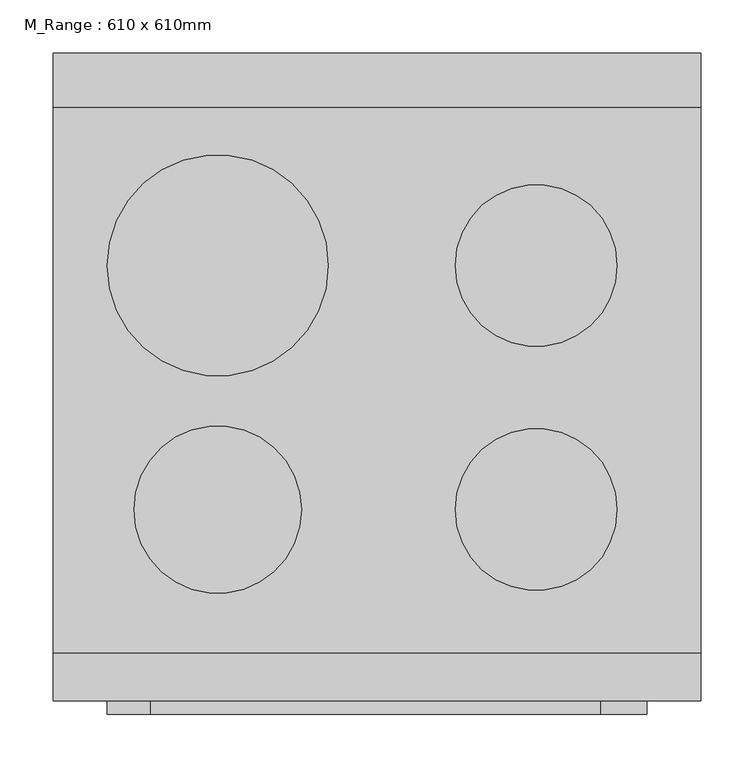
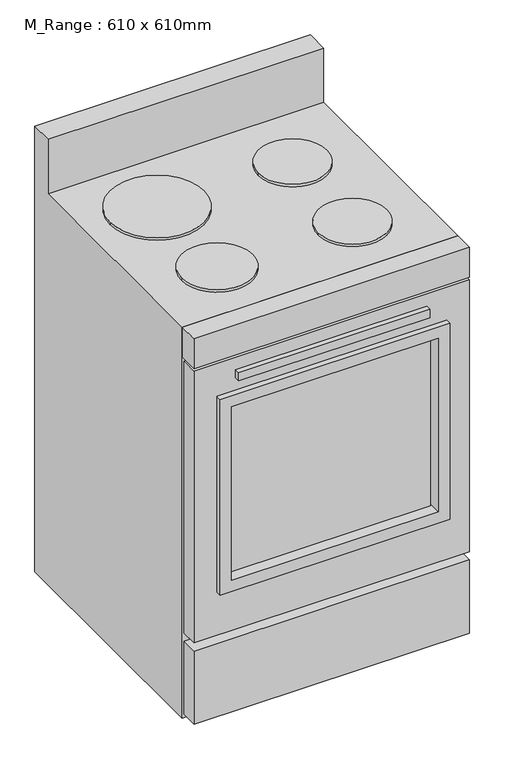
"""IFC4 building model written with IfcOpenShell, lengths in millimetres: proxy geometry, M_Range : 610 x 610mm."""

from ifc_helpers import new_model, si_unit, point, frame, frame_2d, origin, place, context, project, spatial, polyline, circle_curve, trimmed, segment, composite_curve, outline, extrude, faceted_brep, source, transform, mapped, element, save


def m_range_610_x_610mm_0f77da38(model_context):
    return source(origin(), model_context, "Body", "SolidModel", [
        faceted_brep([(610.0, 610.0, 1041.4), (610.0, 559.2, 1041.4), (610.0, 559.2, 914.4), (610.0, 45.0, 914.4), (610.0, 45.0, 0.0), (610.0, 610.0, 0.0), (0.0, 559.2, 914.4), (0.0, 559.2, 1041.4), (0.0, 610.0, 1041.4), (0.0, 610.0, 0.0), (0.0, 45.0, 0.0), (0.0, 45.0, 914.4), (584.6, 45.0, 889.2220355), (584.6, 45.0, 254.0), (25.4, 45.0, 254.0), (25.4, 45.0, 889.2220355), (25.4, 584.6, 889.2220355), (584.6, 584.6, 889.2220355), (25.4, 584.6, 254.0), (584.6, 584.6, 254.0)], [[[0, 1, 2, 3, 4, 5]], [[6, 7, 8, 9, 10, 11]], [[8, 0, 5, 9]], [[1, 0, 8, 7]], [[2, 1, 7, 6]], [[3, 11, 10, 4], [12, 13, 14, 15]], [[9, 5, 4, 10]], [[11, 3, 2, 6]], [[12, 15, 16, 17]], [[15, 14, 18, 16]], [[14, 13, 19, 18]], [[13, 12, 17, 19]], [[17, 16, 18, 19]]]),
        extrude(outline(polyline([(515.325, -12.7), (91.687309, -12.7), (91.687309, 0.0), (515.325, 0.0), (515.325, -12.7)])), frame((0.0, 0.0, 791.2768639), z_axis=(0.0, 0.0, 1.0), x_axis=(1.0, 0.0, 0.0)), (0.0, 0.0, 1.0), 19.05),
        extrude(outline(polyline([(531.2, 12.7), (76.2, 12.7), (76.2, 19.05), (531.2, 19.05), (531.2, 12.7)])), frame((0.0, 0.0, 330.2), z_axis=(0.0, 0.0, 1.0), x_axis=(1.0, 0.0, 0.0)), (0.0, 0.0, 1.0), 406.4),
        extrude(outline(polyline([(610.0, 0.0), (0.0, 0.0), (0.0, 45.0), (610.0, 45.0), (610.0, 0.0)])), frame((0.0, 0.0, 844.7720355), z_axis=(0.0, 0.0, 1.0), x_axis=(1.0, 0.0, 0.0)), (0.0, 0.0, 1.0), 69.6279645),
        extrude(outline(polyline([(762.0, 559.2), (762.0, 50.8), (304.8, 50.8), (304.8, 559.2), (762.0, 559.2)]), holes=[polyline([(736.6, 533.8), (330.2, 533.8), (330.2, 76.2), (736.6, 76.2), (736.6, 533.8)])]), frame((0.0, -12.7, 0.0), z_axis=(0.0, 1.0, 0.0), x_axis=(0.0, 0.0, 1.0)), (0.0, 0.0, 1.0), 38.1),
        extrude(outline(composite_curve([segment(trimmed(circle_curve(frame_2d((155.0, 410.0)), 104.2), [point((50.8, 410.0))], [point((259.2, 410.0))], False, "CARTESIAN"), True, "CONTINUOUS"), segment(trimmed(circle_curve(frame_2d((155.0, 410.0)), 104.2), [point((259.2, 410.0))], [point((50.8, 410.0))], False, "CARTESIAN"), True, "CONTINUOUS")], self_intersect=False)), frame((0.0, 0.0, 914.4), z_axis=(0.0, 0.0, 1.0), x_axis=(1.0, 0.0, 0.0)), (0.0, 0.0, 1.0), 6.35),
        extrude(outline(composite_curve([segment(trimmed(circle_curve(frame_2d((455.0, 410.0)), 76.2), [point((378.8, 410.0))], [point((531.2, 410.0))], False, "CARTESIAN"), True, "CONTINUOUS"), segment(trimmed(circle_curve(frame_2d((455.0, 410.0)), 76.2), [point((531.2, 410.0))], [point((378.8, 410.0))], False, "CARTESIAN"), True, "CONTINUOUS")], self_intersect=False)), frame((0.0, 0.0, 914.4), z_axis=(0.0, 0.0, 1.0), x_axis=(1.0, 0.0, 0.0)), (0.0, 0.0, 1.0), 6.35),
        extrude(outline(composite_curve([segment(trimmed(circle_curve(frame_2d((455.0, 180.0)), 76.2), [point((378.8, 180.0))], [point((531.2, 180.0))], False, "CARTESIAN"), True, "CONTINUOUS"), segment(trimmed(circle_curve(frame_2d((455.0, 180.0)), 76.2), [point((531.2, 180.0))], [point((378.8, 180.0))], False, "CARTESIAN"), True, "CONTINUOUS")], self_intersect=False)), frame((0.0, 0.0, 914.4), z_axis=(0.0, 0.0, 1.0), x_axis=(1.0, 0.0, 0.0)), (0.0, 0.0, 1.0), 6.35),
        extrude(outline(composite_curve([segment(trimmed(circle_curve(frame_2d((155.0, 180.0)), 78.8), [point((76.2, 180.0))], [point((233.8, 180.0))], False, "CARTESIAN"), True, "CONTINUOUS"), segment(trimmed(circle_curve(frame_2d((155.0, 180.0)), 78.8), [point((233.8, 180.0))], [point((76.2, 180.0))], False, "CARTESIAN"), True, "CONTINUOUS")], self_intersect=False)), frame((0.0, 0.0, 914.4), z_axis=(0.0, 0.0, 1.0), x_axis=(1.0, 0.0, 0.0)), (0.0, 0.0, 1.0), 6.35),
        extrude(outline(polyline([(838.4220355, 610.0), (838.4220355, 0.0), (203.2, 0.0), (203.2, 610.0), (838.4220355, 610.0)]), holes=[polyline([(762.0, 559.2), (304.8, 559.2), (304.8, 50.8), (762.0, 50.8), (762.0, 559.2)])]), frame((0.0, 0.0, 0.0), z_axis=(0.0, 1.0, 0.0), x_axis=(0.0, 0.0, 1.0)), (0.0, 0.0, 1.0), 38.1),
        extrude(outline(polyline([(610.0, 0.0), (0.0, 0.0), (0.0, 38.1), (610.0, 38.1), (610.0, 0.0)])), frame((0.0, 0.0, 12.7), z_axis=(0.0, 0.0, 1.0), x_axis=(1.0, 0.0, 0.0)), (0.0, 0.0, 1.0), 171.45),
    ])


if __name__ == "__main__":
    model = new_model("IFC4")
    model_context = context("Model", 3, world=origin())
    ifc_project = project(units=[si_unit("LENGTHUNIT", "METRE", prefix="MILLI")], contexts=[model_context])
    site = spatial("IfcSite", under=ifc_project)
    building = spatial("IfcBuilding", under=site)
    placement = place(None, origin())
    m_range_610_x_610mm_shape = m_range_610_x_610mm_0f77da38(model_context)
    element("IfcBuildingElementProxy", 1, Name="M_Range : 610 x 610mm", ObjectType="M_Range : 610 x 610mm", at=placement, inside=building, context=model_context, shape_type="MappedRepresentation", body=[
        mapped(m_range_610_x_610mm_shape, transform((0.0, 0.0, 0.0), x_axis=(1.0, 0.0, 0.0), y_axis=(0.0, 1.0, 0.0), z_axis=(0.0, 0.0, 1.0))),
    ])
    save(model, "model.ifc")

# Revit data of these elements
# Project information
#   Project Issue Date = "05/02/2018"
#   Project Status = "Project Status"
#   Client Name = "Owner"
#   Project Address = "MADISON, WI"
#   Project Name = "335 WEST LAKESIDE STREET"
#   Project Number = "Project Number"
# Type "M_Range : 610 x 610mm"
#   Depth = 2' - 0.01575"
#   Width = 2' - 0.01575"
#   Burner Material = Steel, Chrome Plated
#   Range Material = Steel, Paint Finish, Ivory, Matte
# Element 1 (IfcBuildingElementProxy, "M_Range : 610 x 610mm")
#   Materials on its faces: "Steel, Paint Finish, Ivory, Matte", "Steel, Chrome Plated", "EXISTING WINDOW"
# Materials
#   "Steel, Chrome Plated": class "Metal", colour RGB 244 244 244, transparency 0, Description = "Chromiuim plated steel", Cost = 0
#   "Steel, Paint Finish, Ivory, Matte": class "Metal", colour RGB 247 247 239, transparency 0, Description = "Steel, paint finish, ivory, matte", Cost = 0
#   "EXISTING WINDOW": class "Glass", colour RGB 218 227 224, transparency 0.85, Description = "Soda Lime Glass", Cost = 0
